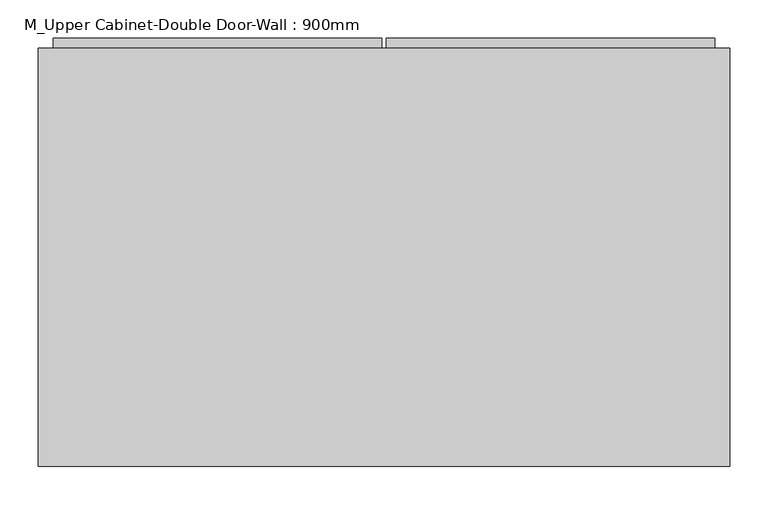
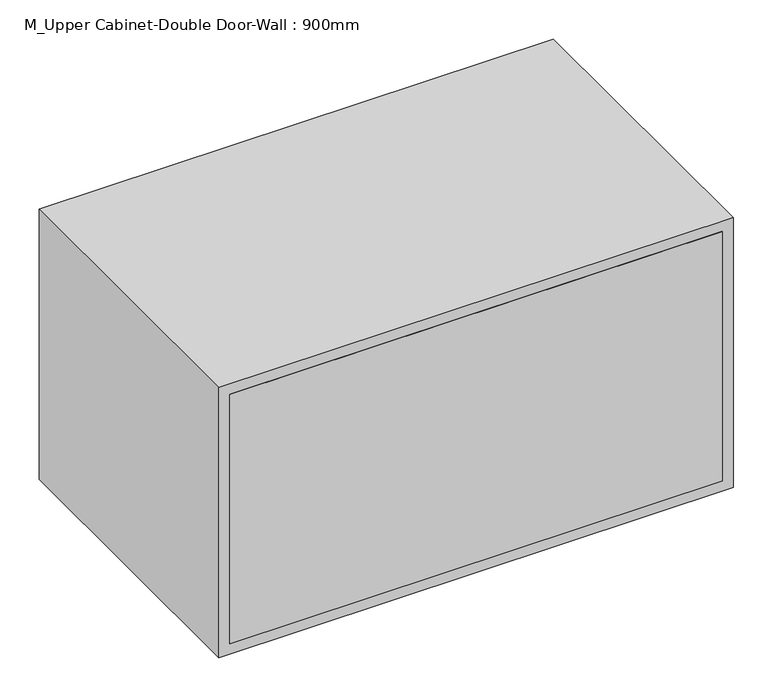
"""IFC4 building model written with IfcOpenShell, lengths in millimetres: furniture geometry, M_Upper Cabinet-Double Door-Wall : 900mm."""

from ifc_helpers import new_model, si_unit, frame, origin, place, context, project, spatial, polyline, outline, extrude, source, transform, mapped, element, save


def m_upper_cabinet_double_door_wall_900mm_7c618084(model_context):
    return source(origin(), model_context, "Body", "SweptSolid", [
        extrude(outline(polyline([(32.9461628, 645.2), (460.7211628, 645.2), (460.7211628, 613.45), (32.9461628, 613.45), (32.9461628, 645.2)])), frame((0.0, 0.0, 119.05), z_axis=(0.0, 0.0, 1.0), x_axis=(1.0, 0.0, 0.0)), (0.0, 0.0, 1.0), 461.9),
        extrude(outline(polyline([(-401.1788372, 645.2), (26.5961628, 645.2), (26.5961628, 613.45), (-401.1788372, 613.45), (-401.1788372, 645.2)])), frame((0.0, 0.0, 119.05), z_axis=(0.0, 0.0, 1.0), x_axis=(1.0, 0.0, 0.0)), (0.0, 0.0, 1.0), 461.9),
        extrude(outline(polyline([(460.7211628, 87.5), (-401.1788372, 87.5), (-401.1788372, 106.55), (460.7211628, 106.55), (460.7211628, 87.5)])), frame((0.0, 0.0, 119.05), z_axis=(0.0, 0.0, 1.0), x_axis=(1.0, 0.0, 0.0)), (0.0, 0.0, 1.0), 461.9),
        extrude(outline(polyline([(600.0, -420.2288372), (100.0, -420.2288372), (100.0, 479.7711628), (600.0, 479.7711628), (600.0, -420.2288372)]), holes=[polyline([(580.95, -401.1788372), (580.95, 460.7211628), (119.05, 460.7211628), (119.05, -401.1788372), (580.95, -401.1788372)])]), frame((0.0, 87.5, 0.0), z_axis=(0.0, 1.0, 0.0), x_axis=(0.0, 0.0, 1.0)), (0.0, 0.0, 1.0), 545.0),
    ])


if __name__ == "__main__":
    model = new_model("IFC4")
    model_context = context("Model", 3, world=origin())
    ifc_project = project(units=[si_unit("LENGTHUNIT", "METRE", prefix="MILLI")], contexts=[model_context])
    site = spatial("IfcSite", under=ifc_project)
    building = spatial("IfcBuilding", under=site)
    placement = place(None, origin())
    m_upper_cabinet_double_door_wall_900mm_shape = m_upper_cabinet_double_door_wall_900mm_7c618084(model_context)
    element("IfcFurniture", 1, ObjectType="M_Upper Cabinet-Double Door-Wall : 900mm", at=placement, inside=building, context=model_context, shape_type="MappedRepresentation", body=[
        mapped(m_upper_cabinet_double_door_wall_900mm_shape, transform((0.0, 0.0, 0.0), x_axis=(1.0, 0.0, 0.0), y_axis=(0.0, 1.0, 0.0), z_axis=(0.0, 0.0, 1.0))),
    ])
    save(model, "model.ifc")

# Revit data of these elements
# Type "M_Upper Cabinet-Double Door-Wall : 900mm"
#   COBie.Type.CreatedBy = "design@eagle.com"
#   COBie.Type.CreatedOn = "2016-09-01T06:50:21"
#   COBie.Type.Name = "Casework_M_Upper Cabinet-Double Door-Wall_900mm"
#   COBie.Type.Category = "23-40 35 17 47 11 : Kitchen Casework"
#   COBie.Type.Description = ""
#   COBie.Type.Manufacturer = ""
#   COBie.Type.ModelNumber = ""
#   COBie.Type.ReplacementCost = 0
#   Depth = 545 mm
#   Height = 500 mm
#   Top Of Cabinet = 600 mm
#   Width = 900 mm
#   COBie.Type = no
#   Cabinet Material = Door - Panel
#   Door/Drawer Material = Door - Panel
#   Handle Material = Cabinets - Handles
# Element 1 (IfcFurniture, "M_Upper Cabinet-Double Door-Wall : 900mm")
#   Materials on its faces: "Door - Panel"
# Materials
#   "Door - Panel": class "Wood", colour RGB 210 159 95, transparency 0
#   "Cabinets - Handles": class "Metal", colour RGB 57 57 57, transparency 0
